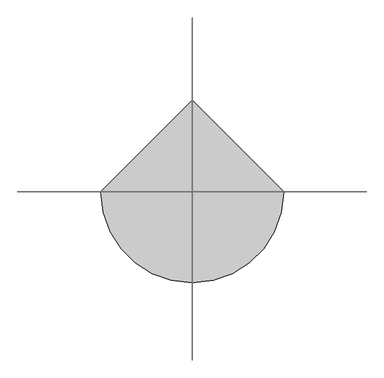
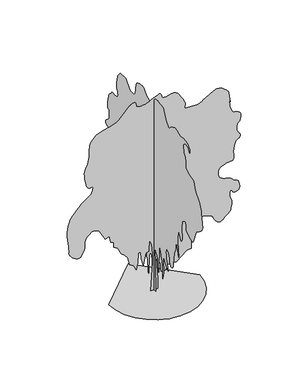
"""IFC4 building model written with IfcOpenShell, lengths in millimetres: geographic element geometry, RPC 木 - 落葉樹 : キングサリ - 5.5 メートル."""

from ifc_helpers import new_model, si_unit, origin, place, context, project, spatial, triangles, source, transform, mapped, element, save


def geographic_element_a00e3d8d(model_context):
    return source(origin(), model_context, "Body", "Tessellation", [
        triangles([(-0.0021492, 84.2526244, 0.0017055), (-0.0021492, -79.7118133, 0.0017055), (-0.0021492, -55.1171344, 770.634066), (-0.0021492, -30.52271, 1205.1392303), (-0.0021492, -128.9011709, 1090.3649134), (-0.0021492, -161.6941638, 983.7871164), (-0.0021492, -161.6941638, 778.8331295), (-0.0021492, -202.6851937, 614.866975), (-0.0021492, -227.2798771, 1410.0957607), (-0.0021492, -292.8648455, 1254.3285244), (-0.0021492, -391.2435608, 934.5977497), (-0.0021492, -407.6416878, 557.4810519), (-0.0021492, -448.631991, 754.2384825), (-0.0021492, -424.0373076, 1123.1586239), (-0.0021492, -399.4426243, 1229.73395), (-0.0021492, -563.406308, 1024.7799631), (-0.0021492, -645.3893852, 910.0031027), (-0.0021492, -571.6053715, 1164.1489271), (-0.0021492, -566.3701896, 1202.7023878), (-0.0021492, -561.3514189, 1240.6803749), (-0.0021492, -556.7629998, 1277.5125744), (-0.0021492, -552.8188002, 1312.6235126), (-0.0021492, -549.7352311, 1345.4427303), (-0.0021492, -547.7261968, 1375.3897396), (-0.0021492, -547.0106881, 1401.8966972), (-0.0021492, -548.2049103, 1425.0577835), (-0.0021492, -551.5507453, 1445.6369053), (-0.0021492, -556.6891671, 1464.0644142), (-0.0021492, -563.2636931, 1480.7706619), (-0.0021492, -570.9127902, 1496.1886162), (-0.0021492, -579.2773596, 1510.7457218), (-0.0021492, -588.000955, 1524.870005), (-0.0021492, -615.9185823, 1493.2475166), (-0.0021492, -642.6878059, 1461.6276443), (-0.0021492, -667.1627655, 1430.0051559), (-0.0021492, -688.1977461, 1398.3828129), (-0.0021492, -704.6417278, 1366.7627953), (-0.0021492, -715.3489231, 1335.1404522), (-0.0021492, -719.1734716, 1303.5179638), (-0.0021492, -720.8463346, 1273.0922047), (-0.0021492, -725.5315138, 1244.8155876), (-0.0021492, -732.7248247, 1218.3341372), (-0.0021492, -741.92717, 1193.2836313), (-0.0021492, -752.6342926, 1169.3103127), (-0.0021492, -764.3473131, 1146.0549734), (-0.0021492, -776.5592857, 1123.1586239), (-0.0021492, -799.2416948, 1123.4208899), (-0.0021492, -820.9921841, 1125.2619112), (-0.0021492, -840.8787609, 1130.2577545), (-0.0021492, -857.9695055, 1139.9845591), (-0.0021492, -871.3299545, 1156.0211529), (-0.0021492, -880.0306589, 1179.9486895), (-0.0021492, -883.1370827, 1213.3382938), (-0.0021492, -884.8100183, 1255.5711811), (-0.0021492, -889.4951975, 1304.2589069), (-0.0021492, -896.6885084, 1358.3243568), (-0.0021492, -905.890781, 1416.6931778), (-0.0021492, -916.5979763, 1478.2854939), (-0.0021492, -928.3109241, 1542.0320389), (-0.0021492, -940.5255129, 1606.8530823), (-0.0021492, -1006.1104631, 1762.6177025), (-0.0021492, -1030.7051828, 2041.3582466), (-0.0021492, -1137.2829798, 1615.049675), (-0.0021492, -1096.2901331, 2033.1591831), (-0.0021492, -1120.8847801, 2385.683741), (-0.0021492, -1260.2563602, 2139.7369801), (-0.0021492, -1270.7241806, 2153.8612633), (-0.0021492, -1280.7616493, 2168.4185143), (-0.0021492, -1289.9410309, 2183.833707), (-0.0021492, -1297.8295029, 2200.5425709), (-0.0021492, -1303.9940975, 2218.9700798), (-0.0021492, -1308.0095501, 2239.5492016), (-0.0021492, -1309.4456543, 2262.7104332), (-0.0021492, -1307.6275967, 2290.0779488), (-0.0021492, -1302.9424175, 2322.0339924), (-0.0021492, -1296.5385933, 2357.1449306), (-0.0021492, -1289.5590775, 2393.9769848), (-0.0021492, -1283.1526371, 2431.0969574), (-0.0021492, -1278.467458, 2467.0685989), (-0.0021492, -1276.6520164, 2500.4581306), (-0.0021492, -1277.8461296, 2532.7959824), (-0.0021492, -1281.1946171, 2566.4378242), (-0.0021492, -1286.3329662, 2601.1438454), (-0.0021492, -1292.9049488, 2636.6899315), (-0.0021492, -1300.5540459, 2672.8984772), (-0.0021492, -1308.9186516, 2709.5395546), (-0.0021492, -1317.642247, 2746.4099785), (-0.0021492, -1349.0965771, 2763.5973015), (-0.0021492, -1379.5477707, 2778.4931946), (-0.0021492, -1407.98993, 2788.7803574), (-0.0021492, -1433.4223892, 2792.1923584), (-0.0021492, -1454.8366344, 2786.4377678), (-0.0021492, -1471.2349068, 2769.1992851), (-0.0021492, -1481.6059307, 2738.2107697), (-0.0021492, -1484.4043064, 2701.9007767), (-0.0021492, -1481.8937038, 2669.6135033), (-0.0021492, -1478.8100258, 2640.331279), (-0.0021492, -1479.8871403, 2613.0602692), (-0.0021492, -1489.8533924, 2586.7825127), (-0.0021492, -1513.4448303, 2560.530336), (-0.0021492, -1555.3924152, 2533.2517685), (-0.0021492, -1606.8990097, 2505.0720932), (-0.0021492, -1655.2531803, 2478.4681938), (-0.0021492, -1699.3015091, 2456.025087), (-0.0021492, -1737.903368, 2440.3222664), (-0.0021492, -1769.9078098, 2433.9411152), (-0.0021492, -1794.1663582, 2439.4615631), (-0.0021492, -1809.5357689, 2459.4679001), (-0.0021492, -1957.1037964, 2820.1761154), (-0.0021492, -2096.4729057, 2918.565168), (-0.0021492, -2133.9034698, 2947.2108032), (-0.0021492, -2168.0339447, 2976.9770096), (-0.0021492, -2197.5760368, 3008.067263), (-0.0021492, -2221.2388367, 3040.5580124), (-0.0021492, -2237.731144, 3074.6530243), (-0.0021492, -2245.7621944, 3110.4540367), (-0.0021492, -2244.0409332, 3148.1136566), (-0.0021492, -2235.2459759, 3194.9401588), (-0.0021492, -2223.8691994, 3254.6760475), (-0.0021492, -2211.3439465, 3322.1530334), (-0.0021492, -2199.1064667, 3392.2016647), (-0.0021492, -2188.5902481, 3459.6786507), (-0.0021492, -2181.2289242, 3519.4145393), (-0.0021492, -2178.455983, 3566.2154617), (-0.0021492, -2170.3281361, 3608.6878693), (-0.0021492, -2147.5744377, 3658.060437), (-0.0021492, -2112.6316578, 3713.1367264), (-0.0021492, -2067.93395, 3772.8220367), (-0.0021492, -2015.9257874, 3835.9446373), (-0.0021492, -1959.038998, 3901.3845383), (-0.0021492, -1899.7154388, 3967.9447197), (-0.0021492, -1842.3295521, 4197.493499), (-0.0021492, -1629.1739582, 4246.6878799), (-0.0021492, -1457.0138271, 4328.6532257), (-0.0021492, -1458.3505188, 4335.1970123), (-0.0021492, -1461.6963902, 4352.7409996), (-0.0021492, -1466.0480141, 4378.3568779), (-0.0021492, -1470.3971672, 4408.9634399), (-0.0021492, -1473.7428932, 4441.6067963), (-0.0021492, -1475.0823463, 4473.206321), (-0.0021492, -1473.409338, 4500.8337044), (-0.0021492, -1467.7438408, 4526.8568253), (-0.0021492, -1458.2079403, 4555.4518822), (-0.0021492, -1445.4434578, 4586.2110512), (-0.0021492, -1430.0994816, 4618.7018005), (-0.0021492, -1412.8176876, 4652.465728), (-0.0021492, -1394.2476002, 4687.1208801), (-0.0021492, -1375.0306046, 4722.1832748), (-0.0021492, -1342.2369667, 4918.9358002), (-0.0021492, -1448.8147636, 5009.1256439), (-0.0021492, -1579.9871349, 4984.5283081), (-0.0021492, -1653.7686779, 4877.9400467), (-0.0021492, -1653.7686779, 4976.32939), (-0.0021492, -1538.9942883, 5082.8914902), (-0.0021492, -1350.4360302, 5107.488826), (-0.0021492, -1202.86793, 5074.692572), (-0.0021492, -1055.2998299, 5156.6834976), (-0.0021492, -948.7220329, 5164.8824158), (-0.0021492, -940.8820318, 5161.1390396), (-0.0021492, -920.1373678, 5151.1070938), (-0.0021492, -890.6410578, 5136.4911255), (-0.0021492, -856.5588358, 5118.9980072), (-0.0021492, -822.0437914, 5100.3340302), (-0.0021492, -791.2591152, 5082.280481), (-0.0021492, -768.3627657, 5066.4936539), (-0.0021492, -752.5401123, 5050.8591431), (-0.0021492, -739.1542288, 5033.7991379), (-0.0021492, -726.6289759, 5017.8844116), (-0.0021492, -713.388287, 5005.688063), (-0.0021492, -697.8532614, 4999.805864), (-0.0021492, -678.4454344, 5002.8359116), (-0.0021492, -653.5859053, 5017.2989822), (-0.0021492, -627.152853, 5039.5790176), (-0.0021492, -603.7294644, 5064.0234558), (-0.0021492, -582.8141713, 5090.2247635), (-0.0021492, -563.9079125, 5117.8777267), (-0.0021492, -546.5090836, 5146.6253906), (-0.0021492, -530.1109202, 5176.0608032), (-0.0021492, -514.2169413, 5205.8775879), (-0.0021492, -415.8382442, 5410.8290314), (-0.0021492, -169.8924643, 5451.8247849), (-0.0021492, -163.845268, 5451.6718872), (-0.0021492, -147.6161895, 5450.6789246), (-0.0021492, -124.0728773, 5447.9540909), (-0.0021492, -96.0842423, 5442.6323227), (-0.0021492, -66.5181782, 5433.8985535), (-0.0021492, -38.242574, 5420.8359787), (-0.0021492, -14.1260636, 5402.6301132), (-0.0021492, 3.3458591, 5384.2457703), (-0.0021492, 15.2248417, 5370.0373352), (-0.0021492, 23.9488607, 5358.0956223), (-0.0021492, 31.9557666, 5346.6114395), (-0.0021492, 41.6836385, 5333.6761826), (-0.0021492, 55.5706315, 5317.4312439), (-0.0021492, 76.0543103, 5296.0418518), (-0.0021492, 97.1353591, 5271.2921997), (-0.0021492, 113.1971422, 5247.5349289), (-0.0021492, 127.251426, 5226.7827072), (-0.0021492, 142.3092006, 5211.0464584), (-0.0021492, 161.3827366, 5202.3638489), (-0.0021492, 187.4830512, 5202.6946426), (-0.0021492, 223.6221243, 5214.0770874), (-0.0021492, 264.3514152, 5233.7851868), (-0.0021492, 302.4974698, 5257.3895599), (-0.0021492, 338.4919115, 5284.2018768), (-0.0021492, 372.7676173, 5313.5861298), (-0.0021492, 405.7523409, 5344.9307281), (-0.0021492, 437.8764338, 5377.549086), (-0.0021492, 469.5676317, 5410.8290314), (-0.0021492, 492.4664884, 5419.4866425), (-0.0021492, 515.7217913, 5427.329187), (-0.0021492, 539.6951826, 5433.618338), (-0.0021492, 564.7456521, 5437.5396103), (-0.0021492, 591.2271389, 5438.3035172), (-0.0021492, 619.503756, 5435.1205719), (-0.0021492, 649.9294424, 5427.227449), (-0.0021492, 681.4067362, 5417.9076691), (-0.0021492, 712.0260155, 5409.8616486), (-0.0021492, 740.9213448, 5401.4080948), (-0.0021492, 767.2373257, 5390.7895569), (-0.0021492, 790.1107115, 5376.3014877), (-0.0021492, 808.683415, 5356.2364334), (-0.0021492, 822.0921896, 5328.8381058), (-0.0021492, 831.6764883, 5297.4679276), (-0.0021492, 839.5394531, 5266.5052826), (-0.0021492, 845.9687845, 5235.9240097), (-0.0021492, 851.252401, 5205.5973724), (-0.0021492, 855.6727707, 5175.5259521), (-0.0021492, 859.5227537, 5145.5556885), (-0.0021492, 863.0824928, 5115.6877441), (-0.0021492, 868.5086151, 5085.9982773), (-0.0021492, 874.8667299, 5057.4029297), (-0.0021492, 883.0887571, 5030.9469864), (-0.0021492, 894.1065439, 5007.6995682), (-0.0021492, 908.8546989, 4988.7803741), (-0.0021492, 928.2625986, 4975.2085281), (-0.0021492, 953.2646336, 4968.1298904), (-0.0021492, 983.5707052, 4964.7946289), (-0.0021492, 1017.0341423, 4962.6302261), (-0.0021492, 1051.7859455, 4962.7319641), (-0.0021492, 1085.9648912, 4966.2968628), (-0.0021492, 1117.7070671, 4974.4446213), (-0.0021492, 1145.1459446, 4988.3478424), (-0.0021492, 1166.417684, 5009.1256439), (-0.0021492, 1187.9516893, 5037.6186722), (-0.0021492, 1215.2250973, 5071.5857849), (-0.0021492, 1244.9327316, 5107.4126678), (-0.0021492, 1273.7822788, 5141.5326782), (-0.0021492, 1298.4736496, 5170.3315018), (-0.0021492, 1315.7070454, 5190.2436584), (-0.0021492, 1322.1822315, 5197.6786697), (-0.0021492, 1576.3282013, 5181.2802521), (-0.0021492, 1674.7067894, 5058.2941544), (-0.0021492, 1679.9878624, 5049.3057495), (-0.0021492, 1685.3427681, 5039.1209061), (-0.0021492, 1690.8402523, 5026.4658646), (-0.0021492, 1696.5540024, 5010.1691849), (-0.0021492, 1702.550584, 4988.9844315), (-0.0021492, 1708.9087715, 4961.7134216), (-0.0021492, 1715.6971653, 4927.1347183), (-0.0021492, 1722.2461842, 4888.9655365), (-0.0021492, 1727.9346451, 4851.6622902), (-0.0021492, 1732.9075974, 4815.0467926), (-0.0021492, 1737.3050034, 4779.0420135), (-0.0021492, 1741.2720577, 4743.4447678), (-0.0021492, 1744.9541004, 4708.1530266), (-0.0021492, 1748.4909485, 4672.9888939), (-0.0021492, 1731.0895397, 4648.3406891), (-0.0021492, 1714.6938835, 4623.4122688), (-0.0021492, 1700.3047909, 4597.923999), (-0.0021492, 1688.927869, 4571.5442139), (-0.0021492, 1681.5665451, 4544.0444389), (-0.0021492, 1679.2239555, 4515.0930084), (-0.0021492, 1682.9058529, 4484.4355774), (-0.0021492, 1691.9172215, 4457.546521), (-0.0021492, 1704.7989933, 4438.9587021), (-0.0021492, 1721.4110607, 4426.9911186), (-0.0021492, 1741.6082291, 4419.8869011), (-0.0021492, 1765.2454491, 4415.940049), (-0.0021492, 1792.1827583, 4413.4448524), (-0.0021492, 1822.2749622, 4410.6438606), (-0.0021492, 1851.5776794, 4410.5165428), (-0.0021492, 1877.0101387, 4414.7180305), (-0.0021492, 1899.7154388, 4419.4540787), (-0.0021492, 1920.8445271, 4421.0583412), (-0.0021492, 1941.543409, 4415.787442), (-0.0021492, 1962.9577995, 4399.8985863), (-0.0021492, 1986.2386459, 4369.6483978), (-0.0021492, 2009.8529022, 4339.0165466), (-0.0021492, 2031.6034641, 4320.2758301), (-0.0021492, 2051.6326195, 4307.2641243), (-0.0021492, 2070.0855629, 4293.8451759), (-0.0021492, 2087.1025475, 4273.8059921), (-0.0021492, 2102.8309479, 4241.0097382), (-0.0021492, 2117.4110172, 4189.2942902), (-0.0021492, 2130.4608021, 4132.1300468), (-0.0021492, 2141.5041687, 4085.4564423), (-0.0021492, 2150.5383556, 4046.6762512), (-0.0021492, 2157.5661243, 4013.1925392), (-0.0021492, 2162.5848587, 3982.4330795), (-0.0021492, 2165.5945587, 3951.8012283), (-0.0021492, 2166.6004566, 3918.7503387), (-0.0021492, 2163.9700939, 3888.1437767), (-0.0021492, 2156.60877, 3865.7364235), (-0.0021492, 2145.3032101, 3850.1274925), (-0.0021492, 2130.8427555, 3839.9679382), (-0.0021492, 2114.016893, 3833.907843), (-0.0021492, 2095.6122025, 3830.546711), (-0.0021492, 2076.4181705, 3828.560495), (-0.0021492, 2076.4181705, 3615.4101334), (-0.0021492, 2076.5863289, 3611.7687859), (-0.0021492, 2077.7576237, 3607.2365044), (-0.0021492, 2080.9353367, 3600.9979317), (-0.0021492, 2087.1279819, 3592.1877136), (-0.0021492, 2097.3334637, 3579.9146255), (-0.0021492, 2112.5578251, 3563.3636009), (-0.0021492, 2133.8066734, 3541.6437057), (-0.0021492, 2158.6890209, 3518.82911), (-0.0021492, 2183.2837406, 3498.7640556), (-0.0021492, 2206.2997776, 3480.0997879), (-0.0021492, 2226.4485477, 3461.613707), (-0.0021492, 2242.4392868, 3441.9561859), (-0.0021492, 2252.9809399, 3419.8799171), (-0.0021492, 2256.7799812, 3394.0605629), (-0.0021492, 2250.3277588, 3369.7687317), (-0.0021492, 2232.2566235, 3352.3776421), (-0.0021492, 2204.5071545, 3340.7155632), (-0.0021492, 2169.0142628, 3333.6369255), (-0.0021492, 2127.7108246, 3329.995578), (-0.0021492, 2082.5369831, 3328.6715309), (-0.0021492, 2035.42794, 3328.4677643), (-0.0021492, 2021.5658501, 3329.995578), (-0.0021492, 2008.8497658, 3330.1737648), (-0.0021492, 1998.4277275, 3327.6276993), (-0.0021492, 1991.4508278, 3320.981884), (-0.0021492, 1989.05984, 3308.8869827), (-0.0021492, 1992.4057114, 3289.9677887), (-0.0021492, 2002.6367729, 3262.9008362), (-0.0021492, 2020.3945553, 3234.9679482), (-0.0021492, 2044.3195484, 3213.2224731), (-0.0021492, 2072.5479126, 3195.7802238), (-0.0021492, 2103.2129013, 3180.7573036), (-0.0021492, 2134.4508202, 3166.3198128), (-0.0021492, 2164.4004456, 3150.6091438), (-0.0021492, 2191.195031, 3131.7155296), (-0.0021492, 2214.6668541, 3115.4703003), (-0.0021492, 2235.4115181, 3106.0996513), (-0.0021492, 2252.7161304, 3099.4538361), (-0.0021492, 2265.8627117, 3091.3822357), (-0.0021492, 2274.1329918, 3077.7086517), (-0.0021492, 2276.8092819, 3054.282756), (-0.0021492, 2273.1756374, 3016.9539299), (-0.0021492, 2263.7594971, 2975.5765137), (-0.0021492, 2250.0399857, 2941.9401947), (-0.0021492, 2232.7353733, 2914.7709229), (-0.0021492, 2212.5636395, 2892.7455231), (-0.0021492, 2190.2376766, 2874.6161064), (-0.0021492, 2166.4806965, 2859.0580444), (-0.0021492, 2142.0057369, 2844.7734512), (-0.0021492, 2133.3763218, 2827.178595), (-0.0021492, 2125.6814426, 2809.2779434), (-0.0021492, 2119.8477871, 2790.7918625), (-0.0021492, 2116.8126526, 2771.4654259), (-0.0021492, 2117.5051975, 2750.9678398), (-0.0021492, 2122.8601032, 2729.044178), (-0.0021492, 2133.8066734, 2705.4145157), (-0.0021492, 2153.6932503, 2682.9815826), (-0.0021492, 2182.4714355, 2663.4008011), (-0.0021492, 2215.9807274, 2644.532476), (-0.0021492, 2250.0629494, 2624.2386566), (-0.0021492, 2280.5623959, 2600.3543587), (-0.0021492, 2303.3160942, 2570.74105), (-0.0021492, 2314.1684841, 2533.2517685), (-0.0021492, 2316.6306885, 2491.7827881), (-0.0021492, 2316.7962307, 2450.4565315), (-0.0021492, 2314.3824245, 2407.4087231), (-0.0021492, 2309.1013515, 2360.7784298), (-0.0021492, 2300.6629131, 2308.6964344), (-0.0021492, 2288.7844231, 2249.3015133), (-0.0021492, 2273.1756374, 2180.7272106), (-0.0021492, 2256.9481396, 2122.3126076), (-0.0021492, 2242.7270599, 2087.8459614), (-0.0021492, 2229.5092621, 2067.1472248), (-0.0021492, 2216.2913189, 2050.0334438), (-0.0021492, 2202.0703846, 2026.3248619), (-0.0021492, 2185.8402706, 1985.8337288), (-0.0021492, 2166.6004566, 1918.3849388), (-0.0021492, 2149.5810013, 1842.5205288), (-0.0021492, 2138.873806, 1783.2936207), (-0.0021492, 2131.751857, 1740.2713921), (-0.0021492, 2125.4904659, 1713.0234913), (-0.0021492, 2117.362619, 1701.1195667), (-0.0021492, 2104.6465347, 1704.1318829), (-0.0021492, 2084.617234, 1721.6274719), (-0.0021492, 2060.5012642, 1758.077718), (-0.0021492, 2037.2459976, 1813.4570412), (-0.0021492, 2014.7062397, 1880.5978558), (-0.0021492, 1992.7392666, 1952.324437), (-0.0021492, 1971.2052612, 2021.4716698), (-0.0021492, 1949.9564129, 2080.8665909), (-0.0021492, 1928.8527592, 2123.3388531), (-0.0021492, 1903.2293232, 2154.4825916), (-0.0021492, 1869.4322582, 2184.768243), (-0.0021492, 1828.8239811, 2214.3332989), (-0.0021492, 1782.766618, 2243.3254246), (-0.0021492, 1732.6198242, 2271.8871986), (-0.0021492, 1679.7511036, 2300.1638157), (-0.0021492, 1625.5174953, 2328.2953835), (-0.0021492, 1580.1042789, 2357.6694626), (-0.0021492, 1536.2697453, 2384.1050583), (-0.0021492, 1495.5901062, 2404.6613617), (-0.0021492, 1459.6415737, 2416.3971279), (-0.0021492, 1430.0026852, 2416.3716934), (-0.0021492, 1408.2522686, 2401.6490456), (-0.0021492, 1395.9662453, 2369.285614), (-0.0021492, 1387.7443634, 2327.3633183), (-0.0021492, 1377.3731941, 2285.8715195), (-0.0021492, 1365.2070763, 2244.7360943), (-0.0021492, 1351.607325, 2203.8884422), (-0.0021492, 1336.9304592, 2163.2545853), (-0.0021492, 1321.5380848, 2122.7659229), (-0.0021492, 1305.7867207, 2082.3484772), (-0.0021492, 1125.4248373, 1926.5840023), (-0.0021492, 1107.9776464, 1907.1276318), (-0.0021492, 1091.2458916, 1886.8820652), (-0.0021492, 1075.9503136, 1865.0602867), (-0.0021492, 1062.803805, 1840.8731003), (-0.0021492, 1052.5269613, 1813.5284031), (-0.0021492, 1045.8352913, 1782.242086), (-0.0021492, 1043.4443035, 1746.2221916), (-0.0021492, 1042.7262514, 1711.1596516), (-0.0021492, 1040.7197605, 1682.5468632), (-0.0021492, 1037.6362278, 1659.3170311), (-0.0021492, 1033.6919918, 1640.3853378), (-0.0021492, 1029.1035364, 1624.6823719), (-0.0021492, 1024.0848021, 1611.1308735), (-0.0021492, 1018.8495838, 1598.6540188), (-0.0021492, 871.2815563, 1500.2752853), (-0.0021492, 854.8859728, 1328.1125381), (-0.0021492, 731.9125923, 1270.7241806), (-0.0021492, 699.1188091, 1057.5711302), (-0.0021492, 567.9463288, 1024.7799631), (-0.0021492, 579.9928682, 1019.3537682), (-0.0021492, 590.5345213, 1012.9956533), (-0.0021492, 598.0639309, 1004.7736988), (-0.0021492, 601.0736672, 993.7558393), (-0.0021492, 598.0639309, 979.0076843), (-0.0021492, 587.5222778, 959.5998573), (-0.0021492, 567.9463288, 934.5977497), (-0.0021492, 544.3090725, 908.8801334), (-0.0021492, 522.3905339, 887.4632721), (-0.0021492, 501.9081359, 869.6341278), (-0.0021492, 482.5715618, 854.6720324), (-0.0021492, 464.0956547, 841.8616224), (-0.0021492, 446.1926414, 830.4822298), (-0.0021492, 428.5773648, 819.8234327), (-0.0021492, 416.3169213, 852.4975285), (-0.0021492, 404.2704183, 880.9396877), (-0.0021492, 392.6541942, 900.9204449), (-0.0021492, 381.6821895, 908.2104795), (-0.0021492, 371.5733952, 898.5778553), (-0.0021492, 362.5365921, 867.7931065), (-0.0021492, 354.7933147, 811.6243692), (-0.0021492, 347.289376, 757.5588467), (-0.0021492, 338.9222631, 728.4470335), (-0.0021492, 329.8396053, 713.1030573), (-0.0021492, 320.1840537, 700.3410456), (-0.0021492, 310.0981868, 678.9725098), (-0.0021492, 299.7245649, 637.8141935), (-0.0021492, 289.2083645, 565.6776083), (-0.0021492, 280.100254, 485.3215756), (-0.0021492, 273.5766333, 424.7553597), (-0.0021492, 269.2021002, 380.6815238), (-0.0021492, 266.5488646, 349.8000149), (-0.0021492, 265.1865931, 328.8160123), (-0.0021492, 264.6849704, 314.4268833), (-0.0021492, 264.6136811, 303.3352093), (-0.0021492, 240.0187434, 811.6243692), (-0.0021492, 227.6618305, 844.6574547), (-0.0021492, 214.9461277, 875.6102892), (-0.0021492, 201.5133903, 902.4024038), (-0.0021492, 187.005355, 922.9586346), (-0.0021492, 171.062996, 935.1961143), (-0.0021492, 153.3280502, 937.0371357), (-0.0021492, 133.441982, 926.4012297), (-0.0021492, 115.7070271, 904.2917507), (-0.0021492, 103.9950785, 874.0086428), (-0.0021492, 97.3026454, 836.9141773), (-0.0021492, 94.6257285, 794.3681551), (-0.0021492, 94.9603102, 747.7377892), (-0.0021492, 97.3026454, 698.3804094), (-0.0021492, 100.6487348, 647.6606855), (-0.0021492, 84.2526244, 237.7500047), (88.443575, 0.0002505, 0.0), (-86.3932913, 0.0002505, 0.0), (-44.7656769, 0.0002025, 807.5808661), (-36.4400495, 0.0001919, 1032.3704882), (-69.7422955, 0.0001759, 1307.1158546), (-128.0216733, 0.0001652, 1448.6492214), (-144.6726737, 0.0001865, 1140.603344), (-227.9279117, 0.0001865, 1115.6267435), (-294.532658, 0.0002025, 799.2544847), (-352.8122947, 0.0001919, 999.0699772), (-361.138676, 0.0001812, 1182.2301636), (-427.7421687, 0.0001812, 1182.2301636), (-444.3923879, 0.0001972, 915.8137218), (-486.0217873, 0.0002079, 732.650992), (-552.62528, 0.0002025, 874.1843588), (-660.8581358, 0.0001972, 940.7903223), (-702.4850281, 0.0001812, 1157.2535631), (-785.7412834, 0.0001759, 1257.1626537), (-877.3239201, 0.0001759, 1332.0925278), (-977.2303946, 0.0001599, 1523.5790955), (-1085.4632504, 0.0001599, 1581.8586777), (-1085.4632504, 0.0001492, 1723.3945152), (-1160.3931244, 0.0001492, 1748.3711884), (-1202.0200167, 0.0001386, 1939.857756), (-1318.5792538, 0.0001386, 1889.9045551), (-1468.4390018, 0.0001226, 2172.9737595), (-1502.3251602, 0.0001226, 2194.044421), (-1536.1348698, 0.0001226, 2213.0729107), (-1569.8020008, 0.0001173, 2228.0247597), (-1603.2501045, 0.0001173, 2236.8604122), (-1636.4054935, 0.0001173, 2237.5401672), (-1669.1992767, 0.0001173, 2228.0247597), (-1701.5550053, 0.0001226, 2206.2768139), (-1733.4728245, 0.0001226, 2179.0187393), (-1764.2270519, 0.0001226, 2153.3621658), (-1792.6513344, 0.0001279, 2127.8509323), (-1817.5796093, 0.0001279, 2101.0307671), (-1837.8479942, 0.0001279, 2071.4427475), (-1852.2881012, 0.0001332, 2037.6304218), (-1859.7411346, 0.0001332, 1998.1374836), (-1862.0709343, 0.0001386, 1954.9318359), (-1863.0894768, 0.0001386, 1911.4360897), (-1864.5459286, 0.0001439, 1868.3756367), (-1868.1871307, 0.0001439, 1826.4813915), (-1875.7599243, 0.0001439, 1786.4790367), (-1889.0133305, 0.0001492, 1749.0994869), (-1909.6943356, 0.0001492, 1715.0681339), (-1930.6657299, 0.0001546, 1683.7079842), (-1945.9586918, 0.0001546, 1654.8228287), (-1959.0645779, 0.0001546, 1629.87159), (-1973.4841919, 0.0001546, 1610.3059238), (-1992.7087452, 0.0001599, 1597.5872234), (-2020.2342453, 0.0001599, 1593.1693245), (-2059.5540836, 0.0001599, 1598.5089695), (-2106.0851097, 0.0001546, 1614.4818317), (-2151.452544, 0.0001546, 1639.629134), (-2193.466404, 0.0001546, 1671.9110298), (-2229.9497875, 0.0001492, 1709.2905796), (-2258.7127121, 0.0001492, 1749.7309891), (-2277.5730434, 0.0001439, 1791.1871796), (-2284.3437057, 0.0001439, 1831.6274437), (-2284.0050636, 0.0001439, 1867.2348633), (-2283.6664215, 0.0001386, 1899.3462753), (-2284.3437057, 0.0001386, 1933.6447632), (-2287.0631618, 0.0001332, 1975.8064339), (-2292.8407162, 0.0001332, 2031.5117546), (-2302.6949112, 0.0001279, 2106.4440994), (-2317.6467602, 0.0001226, 2206.2768139), (-2328.3767738, 0.0001119, 2318.4666229), (-2327.0171185, 0.0001066, 2424.8304794), (-2316.773267, 0.0001013, 2522.6006744), (-2300.8512737, 9.59e-05, 2609.0116791), (-2282.4518154, 9.06e-05, 2681.301162), (-2264.7805103, 9.06e-05, 2736.6829559), (-2251.0432674, 8.53e-05, 2772.4075195), (-2228.7606159, 8.53e-05, 2807.0373825), (-2187.9817097, 7.99e-05, 2856.639006), (-2135.6985638, 7.99e-05, 2914.8473717), (-2078.9008678, 7.46e-05, 2975.2457199), (-2024.5781662, 7.46e-05, 3031.4170006), (-1979.7200031, 6.93e-05, 3076.9447449), (-1951.3211552, 6.93e-05, 3105.4377731), (-1924.2821079, 6.4e-05, 3127.0812195), (-1882.8233013, 6.4e-05, 3155.294323), (-1832.9184986, 6.4e-05, 3188.4469505), (-1780.5385563, 5.86e-05, 3224.9610008), (-1731.6521507, 5.86e-05, 3263.2063408), (-1692.2330452, 5.33e-05, 3301.6042877), (-1668.2519508, 5.33e-05, 3338.5511604), (-1656.1647526, 5.33e-05, 3371.3221252), (-1648.0090004, 4.8e-05, 3398.84748), (-1643.1302284, 4.8e-05, 3421.9934509), (-1640.8716454, 4.8e-05, 3441.6762611), (-1640.5814014, 4.8e-05, 3458.7109772), (-1641.5999439, 4.8e-05, 3473.9888237), (-1643.275423, 4.26e-05, 3488.4263145), (-1673.4947994, 4.26e-05, 3483.4864998), (-1703.0598553, 4.26e-05, 3481.1183304), (-1731.3135086, 4.26e-05, 3483.8172935), (-1757.6015842, 4.26e-05, 3494.1809052), (-1781.2668549, 4.26e-05, 3514.75494), (-1801.657616, 4.26e-05, 3548.0604652), (-1818.114315, 3.73e-05, 3596.643837), (-1832.6281094, 3.2e-05, 3658.2386238), (-1846.5615612, 3.2e-05, 3726.3521988), (-1858.3075012, 2.66e-05, 3797.4193726), (-1866.2698059, 2.13e-05, 3867.7226395), (-1868.8440674, 1.6e-05, 3933.671521), (-1864.4263138, 1.6e-05, 3991.625251), (-1851.4147533, 1.07e-05, 4037.891613), (-1831.8515579, 1.07e-05, 4080.6183655), (-1810.1036121, 5.3e-06, 4129.8891953), (-1788.0628063, 5.3e-06, 4185.1439621), (-1767.626263, 0.0, 4245.7710754), (-1750.6832565, -5.3e-06, 4311.2109764), (-1739.1281479, -1.07e-05, 4380.8776543), (-1734.8580597, -1.07e-05, 4454.1856796), (-1735.4895618, -1.6e-05, 4523.8776466), (-1735.828204, -2.13e-05, 4584.5303398), (-1733.5466572, -2.13e-05, 4638.3337418), (-1726.3126511, -2.66e-05, 4687.5028336), (-1711.7987114, -3.2e-05, 4734.1764381), (-1687.670097, -3.2e-05, 4780.5442474), (-1651.6018044, -3.73e-05, 4828.8221146), (-1604.6581581, -3.73e-05, 4875.2410835), (-1551.3057461, -4.26e-05, 4914.6575729), (-1494.3144573, -4.26e-05, 4947.2247711), (-1436.4473499, -4.26e-05, 4973.1208649), (-1380.4746037, -4.26e-05, 4992.421431), (-1329.1617474, -4.8e-05, 5005.3566879), (-1285.2761993, -4.8e-05, 5012.0027939), (-1238.8191513, -4.8e-05, 5019.8197586), (-1181.7285954, -4.8e-05, 5034.7665207), (-1119.6855074, -4.8e-05, 5054.8059952), (-1058.3732615, -4.8e-05, 5077.9260956), (-1003.4674559, -5.33e-05, 5102.03974), (-960.6514647, -5.33e-05, 5125.1604218), (-935.6010315, -5.33e-05, 5145.1993149), (-669.1845171, -6.93e-05, 5428.27099), (-646.0030832, -6.93e-05, 5444.1601364), (-622.8954094, -7.46e-05, 5458.928421), (-599.9329302, -7.46e-05, 5471.5328842), (-577.1894056, -7.46e-05, 5480.8520828), (-554.7387048, -7.46e-05, 5485.7918976), (-532.6495734, -7.46e-05, 5485.2826263), (-510.9984241, -7.46e-05, 5478.2295685), (-495.8275841, -7.46e-05, 5462.4933197), (-489.5407948, -6.93e-05, 5439.0418442), (-486.7500495, -6.93e-05, 5411.3894623), (-482.0648704, -6.93e-05, 5382.9725922), (-470.0972506, -6.93e-05, 5357.3567139), (-445.4618357, -6.4e-05, 5337.9794083), (-402.7655319, -6.4e-05, 5328.3544144), (-352.155358, -6.4e-05, 5326.9794983), (-306.7905398, -6.4e-05, 5329.5258545), (-265.7951679, -6.4e-05, 5335.3568939), (-228.2925333, -6.4e-05, 5343.8104477), (-193.4123586, -6.4e-05, 5354.2249283), (-160.2802058, -6.93e-05, 5365.9381668), (-128.0216733, -6.93e-05, 5378.3129929), (-76.4902348, -6.93e-05, 5408.3594147), (-26.1968067, -6.93e-05, 5436.750705), (21.6206802, -7.46e-05, 5461.7805725), (65.7244948, -7.46e-05, 5481.7688873), (104.8766017, -7.46e-05, 5495.0605179), (137.8389248, -7.46e-05, 5500.0003326), (163.3739486, -7.46e-05, 5494.8826218), (179.7578323, -7.46e-05, 5482.2525787), (188.4231464, -7.46e-05, 5466.2872742), (192.8648993, -7.46e-05, 5447.6994553), (196.5786806, -6.93e-05, 5427.2018692), (203.0594986, -6.93e-05, 5405.5584229), (215.802707, -6.93e-05, 5383.4562836), (238.3035683, -6.93e-05, 5361.6599396), (275.7078986, -6.4e-05, 5352.0099472), (327.5301169, -6.93e-05, 5359.8269119), (388.8194718, -6.93e-05, 5376.0974304), (454.6234131, -6.93e-05, 5391.7575211), (519.9894087, -6.93e-05, 5397.8431961), (579.9673974, -6.93e-05, 5385.2643127), (629.6048836, -6.4e-05, 5345.0074677), (669.510442, -6.4e-05, 5289.625383), (704.1732244, -5.86e-05, 5237.2989258), (734.4639627, -5.86e-05, 5187.5188248), (761.2611643, -5.33e-05, 5139.7758087), (785.4382496, -5.33e-05, 5093.5606064), (807.8660231, -4.8e-05, 5048.3639465), (829.4204487, -4.8e-05, 5003.6765579), (821.0940674, -3.73e-05, 4853.8014038), (1104.1632717, -3.73e-05, 4837.1486412), (1130.9121477, -3.73e-05, 4839.0836975), (1157.5871183, -3.73e-05, 4841.7826607), (1184.116967, -3.73e-05, 4846.1114662), (1210.4304045, -3.73e-05, 4852.8337303), (1236.4509819, -3.73e-05, 4862.7642288), (1262.1075554, -3.73e-05, 4876.6924484), (1287.3260742, -3.73e-05, 4895.433165), (1317.642247, -4.26e-05, 4918.5538467), (1357.5732399, -4.26e-05, 4944.7039948), (1405.5098488, -4.26e-05, 4973.4260788), (1459.8579849, -4.8e-05, 5004.1858292), (1519.0110603, -4.8e-05, 5036.4728119), (1581.3672832, -4.8e-05, 5069.7527573), (1645.3251526, -5.33e-05, 5103.5675537), (1684.4540142, -5.33e-05, 5099.8497574), (1722.8522518, -5.33e-05, 5095.2668976), (1759.7965084, -5.33e-05, 5088.9515854), (1794.5558693, -4.8e-05, 5079.9887604), (1826.3998558, -4.8e-05, 5067.5371948), (1854.6052563, -4.8e-05, 5050.7062454), (1878.441156, -4.8e-05, 5028.6552658), (1900.2145363, -4.8e-05, 5007.1902969), (1922.1329659, -4.26e-05, 4990.5372437), (1943.3232422, -4.26e-05, 4975.3358459), (1962.9120174, -4.26e-05, 4958.2502609), (1980.023037, -4.26e-05, 4935.9196472), (1993.7858597, -3.73e-05, 4905.0075806), (2003.3268471, -3.73e-05, 4862.1276398), (2036.6272854, -2.13e-05, 4620.6877258), (2031.3360386, -2.66e-05, 4643.2226875), (2026.4090137, -2.66e-05, 4661.7340576), (2022.2101421, -2.66e-05, 4672.2502762), (2019.1036457, -2.66e-05, 4670.7480423), (2017.4511303, -2.66e-05, 4653.2296349), (2017.6217594, -2.13e-05, 4615.6717529), (2019.9769936, -2.13e-05, 4554.0766754), (2029.0544918, -1.6e-05, 4483.8245682), (2046.7257969, -1.07e-05, 4423.1715843), (2069.3470905, -5.3e-06, 4372.5514183), (2093.2797867, -5.3e-06, 4332.4216003), (2114.8825378, -5.3e-06, 4303.241114), (2130.5142872, -5.3e-06, 4285.3916222), (2136.5336872, 0.0, 4279.3568161), (2147.5540901, 0.0, 4280.1463028), (2175.7594906, 0.0, 4279.6370316), (2213.8673389, 0.0, 4273.4493279), (2254.597847, 0.0, 4257.2040985), (2290.6661396, 0.0, 4226.5466675), (2314.7948994, 5.3e-06, 4177.0976509), (2319.6964897, 1.07e-05, 4104.5026634), (2308.0217663, 1.07e-05, 4035.0650414), (2289.5025478, 1.6e-05, 3991.3961952), (2267.4871765, 1.6e-05, 3963.6159142), (2245.3242851, 1.6e-05, 3941.794281), (2226.3696281, 2.13e-05, 3916.0257957), (2213.9641354, 2.13e-05, 3876.4308289), (2211.4661774, 2.66e-05, 3813.1044617), (2219.5964951, 2.66e-05, 3747.2826073), (2234.7189732, 3.2e-05, 3702.4170319), (2253.6252319, 3.2e-05, 3671.9886566), (2273.1170654, 3.73e-05, 3649.4284058), (2289.9862392, 3.73e-05, 3628.1416237), (2301.0320766, 3.73e-05, 3601.6601006), (2303.0461979, 4.26e-05, 3563.3383118), (2294.2843781, 4.26e-05, 3529.0395332), (2276.7837021, 4.26e-05, 3512.2341637), (2253.0191643, 4.26e-05, 3502.8382256), (2225.4708458, 4.26e-05, 3490.8197731), (2196.6085087, 4.8e-05, 3466.1206993), (2168.9149956, 4.8e-05, 3418.7340569), (2144.8600685, 5.33e-05, 3338.5511604), (2129.882785, 5.86e-05, 3243.8799042), (2124.958231, 6.4e-05, 3160.2850067), (2125.8545425, 6.93e-05, 3088.6321129), (2128.3549713, 7.46e-05, 3029.812738), (2128.2327404, 7.46e-05, 2984.6669472), (2121.2661598, 7.46e-05, 2954.085965), (2103.2332489, 7.99e-05, 2938.9354362), (2080.3674934, 7.99e-05, 2933.5627991), (2059.9793484, 7.99e-05, 2930.6853584), (2039.4433926, 7.99e-05, 2928.6482735), (2016.1423439, 7.99e-05, 2925.9237305), (1987.4506359, 7.99e-05, 2920.8565979), (1950.7508411, 7.99e-05, 2911.8429039), (1903.4176838, 7.99e-05, 2897.3033844), (1853.5128811, 7.99e-05, 2880.1413506), (1811.035532, 7.99e-05, 2862.9793167), (1776.2786419, 8.53e-05, 2843.7801979), (1749.5298386, 8.53e-05, 2820.5071999), (1731.0818367, 8.53e-05, 2791.0973671), (1721.2276417, 9.06e-05, 2753.565065), (1720.2574974, 9.06e-05, 2705.822049), (1723.6314194, 9.59e-05, 2658.5118553), (1727.8785439, 9.59e-05, 2621.9725159), (1734.8910519, 9.59e-05, 2593.7341232), (1746.5683914, 0.0001013, 2571.3520592), (1764.7947498, 0.0001013, 2552.2802582), (1791.4723366, 0.0001013, 2534.1049141), (1828.4878098, 0.0001013, 2514.3226913), (1873.0047146, 0.0001013, 2496.0453186), (1919.5613205, 0.0001066, 2482.2824959), (1966.1151649, 0.0001066, 2470.414325), (2010.6320698, 0.0001066, 2457.8153847), (2051.0698631, 0.0001066, 2441.8678116), (2085.3913147, 0.0001066, 2419.9518528), (2111.5571594, 0.0001119, 2389.4394711), (2135.6603394, 0.0001119, 2361.7918854), (2163.6951107, 0.0001119, 2345.6508648), (2193.4790485, 0.0001119, 2334.1695889), (2222.8252224, 0.0001119, 2320.5061787), (2249.5485912, 0.0001173, 2297.8085815), (2271.4670208, 0.0001173, 2259.2397148), (2286.3960514, 0.0001226, 2197.9504326), (2290.302063, 0.0001279, 2132.9740208), (2281.9781525, 0.0001279, 2085.908289), (2263.4564632, 0.0001279, 2053.7714424), (2236.7814926, 0.0001332, 2033.5767448), (2203.9877094, 0.0001332, 2022.3374599), (2167.1172855, 0.0001332, 2017.0716476), (2128.209922, 0.0001332, 2014.7876301), (2106.9228493, 0.0001332, 2046.2217579), (2086.3640751, 0.0001279, 2073.5764835), (2067.2591366, 0.0001279, 2092.7782185), (2050.3415646, 0.0001279, 2099.7423283), (2036.3368961, 0.0001279, 2090.3974045), (2025.9709591, 0.0001279, 2060.6643356), (2019.9769936, 0.0001332, 2006.4638649), (2022.332373, 0.0001386, 1947.8938934), (2033.7142365, 0.0001386, 1903.8862598), (2049.9036552, 0.0001439, 1868.6174824), (2066.6760326, 0.0001439, 1836.2617538), (2079.809824, 0.0001439, 1800.9929764), (2085.0756363, 0.0001492, 1756.9878136), (2078.254105, 0.0001492, 1698.4179874), (2066.0701103, 0.0001546, 1638.7047718), (2056.2159153, 0.0001599, 1592.8306824), (2045.923811, 0.0001599, 1557.2946247), (2032.4284138, 0.0001599, 1528.6053875), (2012.9620148, 0.0001652, 1503.2646378), (1984.7566143, 0.0001652, 1477.7762226), (1945.0471195, 0.0001652, 1448.6492214), (1902.3508884, 0.0001705, 1414.6918465), (1865.4804646, 0.0001705, 1379.8609783), (1832.1061935, 0.0001705, 1348.3785976), (1799.8955143, 0.0001759, 1324.4688652), (1766.5212433, 0.0001759, 1312.3587032), (1729.6508194, 0.0001759, 1316.2647148), (1686.9545883, 0.0001705, 1340.416293), (1647.1228626, 0.0001705, 1378.2109337), (1618.067078, 0.0001705, 1418.4780979), (1596.2936977, 0.0001652, 1458.6026836), (1578.309185, 0.0001652, 1495.9567989), (1560.6149162, 0.0001599, 1527.9256325), (1539.7148838, 0.0001599, 1551.881147), (1512.1156963, 0.0001599, 1565.2085312), (1471.7517357, 0.0001599, 1577.5375751), (1418.5698074, 0.0001599, 1596.568681), (1358.1054749, 0.0001546, 1616.7633785), (1295.8943012, 0.0001546, 1632.5885754), (1237.4695244, 0.0001546, 1638.511179), (1188.3667803, 0.0001546, 1628.9957714), (1154.1165453, 0.0001599, 1598.5089695), (1127.3931765, 0.0001599, 1577.4409241), (1098.3373919, 0.0001599, 1588.9960327), (1068.7010468, 0.0001546, 1616.8600296), (1040.2282934, 0.0001546, 1644.7267879), (1014.6711325, 0.0001546, 1656.2792805), (993.7711727, 0.0001546, 1635.211235), (979.2801968, 0.0001599, 1565.2085312), (971.878105, 0.0001652, 1477.5598114), (970.0091057, 0.0001705, 1410.4445766), (972.0716251, 0.0001705, 1357.8941505), (976.4639442, 0.0001759, 1313.9347698), (981.5871054, 0.0001759, 1272.5981941), (985.8343025, 0.0001812, 1227.9132763), (987.6065781, 0.0001812, 1173.9063257), (995.9304159, 0.0002025, 832.5574665), (871.0472683, 0.0002025, 807.5808661), (729.5139742, 0.0002132, 691.0215563), (587.978064, 0.0002185, 591.1150818), (396.4889165, 0.0002185, 599.4414994), (329.8854601, 0.0002185, 557.8146435), (304.9088233, 0.0002238, 457.9055892), (278.3305764, 0.0002238, 452.8104424), (252.8434148, 0.0002238, 449.2405294), (229.5414941, 0.0002238, 448.7312945), (209.5164083, 0.0002238, 452.8104424), (193.8604962, 0.0002238, 463.0032795), (183.6658968, 0.0002238, 480.8451774), (180.024949, 0.0002238, 507.8588264), (179.9037354, 0.0002185, 542.6438035), (179.0540417, 0.0002185, 581.2125612), (176.7483685, 0.0002132, 621.2378071), (172.2579812, 0.0002132, 660.3896324), (164.854872, 0.0002132, 696.3382376), (153.8105607, 0.0002079, 726.7512068), (138.39733, 0.0002079, 749.3012112), (121.7702653, 0.0002079, 768.1132896), (107.3279238, 0.0002079, 788.6720638), (94.705938, 0.0002025, 810.6873625), (83.5404222, 0.0002025, 833.8687963), (73.4672725, 0.0002025, 857.9236507), (64.1223669, 0.0002025, 882.5590656), (55.1413245, 0.0001972, 907.4873405), (63.4669473, 0.0002132, 691.0215563), (88.443575, 0.0002345, 266.4190033), (-1216.0704672, 0.0, 0.0051165), (-1183.9209034, -278.6437659, 0.0051165), (-1092.3612305, -534.53129, 0.0051165), (-948.7220329, -760.3343313, 0.0051165), (-760.3343313, -948.7220329, 0.0051165), (-534.53129, -1092.3612305, 0.0051165), (-278.6437659, -1183.9209034, 0.0051165), (5.32e-05, -1216.0704672, 0.0051165), (278.6437659, -1183.9209034, 0.0051165), (534.53129, -1092.3612305, 0.0051165), (760.3343313, -948.7220329, 0.0051165), (948.7220329, -760.3343313, 0.0051165), (1092.3612305, -534.53129, 0.0051165), (1183.9209034, -278.6437659, 0.0051165), (1216.0704672, 0.0001066, 0.0051165), (-0.0001595, 1216.0704672, 0.0051165)], [[476, 477, 478], [475, 476, 478], [474, 475, 478], [473, 474, 478], [62, 63, 64], [472, 473, 478], [471, 472, 478], [470, 471, 478], [11, 12, 13], [11, 13, 14], [7, 8, 9], [6, 7, 9], [16, 17, 18], [469, 470, 478], [5, 6, 9], [10, 11, 14], [10, 14, 15], [468, 469, 478], [151, 152, 153], [151, 153, 154], [15, 16, 18], [467, 468, 478], [150, 151, 154], [150, 154, 155], [4, 5, 9], [15, 18, 19], [65, 66, 67], [65, 67, 68], [65, 68, 69], [65, 69, 70], [65, 70, 71], [65, 71, 72], [65, 72, 73], [65, 73, 74], [65, 74, 75], [65, 75, 76], [65, 76, 77], [466, 467, 478], [465, 466, 478], [464, 465, 478], [463, 464, 478], [15, 19, 20], [455, 456, 457], [65, 77, 78], [149, 150, 155], [149, 155, 156], [15, 20, 21], [62, 64, 65], [1, 2, 3], [493, 1, 3], [492, 493, 3], [491, 492, 3], [490, 491, 3], [489, 490, 3], [489, 3, 4], [488, 489, 4], [487, 488, 4], [486, 487, 4], [485, 486, 4], [484, 485, 4], [462, 463, 478], [462, 478, 479], [65, 78, 79], [15, 21, 22], [462, 479, 480], [461, 462, 480], [461, 480, 481], [391, 392, 393], [454, 455, 457], [440, 441, 442], [15, 22, 23], [65, 79, 80], [391, 393, 394], [390, 391, 394], [390, 394, 395], [389, 390, 395], [389, 395, 396], [388, 389, 396], [388, 396, 397], [387, 388, 397], [387, 397, 398], [386, 387, 398], [386, 398, 399], [385, 386, 399], [385, 399, 400], [384, 385, 400], [131, 132, 133], [45, 46, 47], [438, 439, 440], [383, 384, 400], [383, 400, 401], [382, 383, 401], [381, 382, 401], [380, 381, 401], [379, 380, 401], [379, 401, 402], [378, 379, 402], [378, 402, 403], [377, 378, 403], [376, 377, 403], [376, 403, 404], [375, 376, 404], [374, 375, 404], [373, 374, 404], [372, 373, 404], [371, 372, 404], [370, 371, 404], [369, 370, 404], [368, 369, 404], [367, 368, 404], [367, 404, 405], [366, 367, 405], [366, 405, 406], [366, 406, 407], [365, 366, 407], [365, 407, 408], [365, 408, 409], [364, 365, 409], [364, 409, 410], [363, 364, 410], [363, 410, 411], [15, 23, 24], [10, 15, 24], [9, 10, 24], [9, 24, 25], [9, 25, 26], [9, 26, 27], [9, 27, 28], [9, 28, 29], [179, 180, 181], [454, 457, 458], [453, 454, 458], [452, 453, 458], [461, 481, 482], [452, 458, 459], [451, 452, 459], [250, 251, 252], [9, 29, 30], [65, 80, 81], [460, 461, 482], [249, 250, 252], [249, 252, 253], [248, 249, 253], [247, 248, 253], [246, 247, 253], [246, 253, 254], [246, 254, 255], [246, 255, 256], [246, 256, 257], [246, 257, 258], [246, 258, 259], [246, 259, 260], [245, 246, 260], [245, 260, 261], [244, 245, 261], [244, 261, 262], [244, 262, 263], [244, 263, 264], [243, 244, 264], [243, 264, 265], [243, 265, 266], [243, 266, 267], [243, 267, 268], [243, 268, 269], [243, 269, 270], [243, 270, 271], [243, 271, 272], [242, 243, 272], [242, 272, 273], [241, 242, 273], [362, 363, 411], [450, 451, 459], [362, 411, 412], [483, 484, 4], [9, 30, 31], [241, 273, 274], [240, 241, 274], [449, 450, 459], [449, 459, 460], [448, 449, 460], [447, 448, 460], [446, 447, 460], [445, 446, 460], [444, 445, 460], [443, 444, 460], [442, 443, 460], [361, 362, 412], [9, 31, 32], [65, 81, 82], [106, 107, 108], [105, 106, 108], [105, 108, 109], [104, 105, 109], [103, 104, 109], [102, 103, 109], [101, 102, 109], [100, 101, 109], [99, 100, 109], [98, 99, 109], [97, 98, 109], [96, 97, 109], [95, 96, 109], [94, 95, 109], [93, 94, 109], [92, 93, 109], [45, 47, 48], [44, 45, 48], [44, 48, 49], [44, 49, 50], [44, 50, 51], [44, 51, 52], [44, 52, 53], [43, 44, 53], [43, 53, 54], [42, 43, 54], [41, 42, 54], [40, 41, 54], [40, 54, 55], [39, 40, 55], [38, 39, 55], [38, 55, 56], [37, 38, 56], [37, 56, 57], [36, 37, 57], [36, 57, 58], [35, 36, 58], [35, 58, 59], [34, 35, 59], [33, 34, 59], [33, 59, 60], [32, 33, 60], [32, 60, 61], [32, 61, 62], [239, 240, 274], [179, 181, 182], [179, 182, 183], [179, 183, 184], [179, 184, 185], [179, 185, 186], [179, 186, 187], [179, 187, 188], [179, 188, 189], [179, 189, 190], [179, 190, 191], [179, 191, 192], [179, 192, 193], [179, 193, 194], [179, 194, 195], [179, 195, 196], [179, 196, 197], [179, 197, 198], [178, 179, 198], [177, 178, 198], [177, 198, 199], [176, 177, 199], [175, 176, 199], [174, 175, 199], [442, 460, 482], [442, 482, 483], [442, 483, 4], [440, 442, 4], [438, 440, 4], [438, 4, 9], [360, 361, 412], [239, 274, 275], [174, 199, 200], [173, 174, 200], [436, 437, 438], [435, 436, 438], [434, 435, 438], [433, 434, 438], [433, 438, 9], [432, 433, 9], [431, 432, 9], [430, 431, 9], [429, 430, 9], [428, 429, 9], [427, 428, 9], [426, 427, 9], [426, 9, 32], [426, 32, 62], [426, 62, 65], [425, 426, 65], [424, 425, 65], [423, 424, 65], [422, 423, 65], [421, 422, 65], [420, 421, 65], [419, 420, 65], [418, 419, 65], [417, 418, 65], [416, 417, 65], [415, 416, 65], [414, 415, 65], [414, 65, 82], [414, 82, 83], [414, 83, 84], [414, 84, 85], [414, 85, 86], [414, 86, 87], [413, 414, 87], [238, 239, 275], [359, 360, 412], [148, 149, 156], [148, 156, 157], [148, 157, 158], [148, 158, 159], [148, 159, 160], [148, 160, 161], [148, 161, 162], [148, 162, 163], [148, 163, 164], [148, 164, 165], [148, 165, 166], [148, 166, 167], [148, 167, 168], [148, 168, 169], [148, 169, 170], [147, 148, 170], [146, 147, 170], [145, 146, 170], [144, 145, 170], [143, 144, 170], [142, 143, 170], [141, 142, 170], [140, 141, 170], [139, 140, 170], [138, 139, 170], [137, 138, 170], [136, 137, 170], [135, 136, 170], [134, 135, 170], [134, 170, 171], [359, 412, 413], [359, 413, 87], [92, 109, 110], [324, 325, 326], [323, 324, 326], [323, 326, 327], [322, 323, 327], [321, 322, 327], [321, 327, 328], [320, 321, 328], [320, 328, 329], [319, 320, 329], [319, 329, 330], [318, 319, 330], [317, 318, 330], [317, 330, 331], [317, 331, 332], [316, 317, 332], [316, 332, 333], [315, 316, 333], [314, 315, 333], [314, 333, 334], [313, 314, 334], [312, 313, 334], [312, 334, 335], [311, 312, 335], [359, 87, 88], [237, 238, 275], [358, 359, 88], [357, 358, 88], [356, 357, 88], [355, 356, 88], [354, 355, 88], [353, 354, 88], [352, 353, 88], [351, 352, 88], [350, 351, 88], [349, 350, 88], [348, 349, 88], [347, 348, 88], [346, 347, 88], [345, 346, 88], [344, 345, 88], [343, 344, 88], [342, 343, 88], [341, 342, 88], [340, 341, 88], [339, 340, 88], [338, 339, 88], [337, 338, 88], [336, 337, 88], [335, 336, 88], [311, 335, 88], [310, 311, 88], [309, 310, 88], [309, 88, 89], [309, 89, 90], [172, 173, 200], [91, 92, 110], [91, 110, 111], [91, 111, 112], [91, 112, 113], [91, 113, 114], [91, 114, 115], [91, 115, 116], [91, 116, 117], [91, 117, 118], [91, 118, 119], [91, 119, 120], [91, 120, 121], [91, 121, 122], [91, 122, 123], [91, 123, 124], [91, 124, 125], [91, 125, 126], [91, 126, 127], [91, 127, 128], [91, 128, 129], [91, 129, 130], [91, 130, 131], [91, 131, 133], [90, 91, 133], [309, 90, 133], [309, 133, 134], [309, 134, 171], [309, 171, 172], [309, 172, 200], [309, 200, 201], [309, 201, 202], [309, 202, 203], [309, 203, 204], [309, 204, 205], [309, 205, 206], [309, 206, 207], [309, 207, 208], [309, 208, 209], [308, 309, 209], [285, 286, 287], [284, 285, 287], [284, 287, 288], [283, 284, 288], [282, 283, 288], [282, 288, 289], [281, 282, 289], [237, 275, 276], [281, 289, 290], [236, 237, 276], [304, 305, 306], [303, 304, 306], [303, 306, 307], [302, 303, 307], [302, 307, 308], [301, 302, 308], [300, 301, 308], [299, 300, 308], [298, 299, 308], [297, 298, 308], [296, 297, 308], [295, 296, 308], [294, 295, 308], [293, 294, 308], [292, 293, 308], [291, 292, 308], [290, 291, 308], [281, 290, 308], [280, 281, 308], [279, 280, 308], [278, 279, 308], [277, 278, 308], [276, 277, 308], [236, 276, 308], [221, 222, 223], [220, 221, 223], [219, 220, 223], [219, 223, 224], [218, 219, 224], [218, 224, 225], [217, 218, 225], [217, 225, 226], [217, 226, 227], [216, 217, 227], [216, 227, 228], [215, 216, 228], [214, 215, 228], [213, 214, 228], [212, 213, 228], [211, 212, 228], [210, 211, 228], [209, 210, 228], [209, 228, 229], [209, 229, 230], [209, 230, 231], [209, 231, 232], [209, 232, 233], [209, 233, 234], [235, 236, 308], [235, 308, 209], [235, 209, 234], [711, 712, 713], [711, 713, 714], [711, 714, 715], [501, 502, 503], [506, 507, 508], [501, 503, 504], [494, 495, 496], [889, 494, 496], [888, 889, 496], [887, 888, 496], [887, 496, 497], [517, 518, 519], [859, 860, 861], [499, 500, 501], [499, 501, 504], [711, 715, 716], [505, 506, 508], [505, 508, 509], [505, 509, 510], [865, 866, 867], [513, 514, 515], [845, 846, 847], [515, 516, 517], [802, 803, 804], [865, 867, 868], [505, 510, 511], [865, 868, 869], [865, 869, 870], [865, 870, 871], [865, 871, 872], [865, 872, 873], [865, 873, 874], [865, 874, 875], [865, 875, 876], [865, 876, 877], [864, 865, 877], [864, 877, 878], [845, 847, 848], [844, 845, 848], [844, 848, 849], [499, 504, 505], [499, 505, 511], [499, 511, 512], [499, 512, 513], [499, 513, 515], [864, 878, 879], [499, 515, 517], [862, 863, 864], [862, 864, 879], [862, 879, 880], [861, 862, 880], [859, 861, 880], [859, 880, 881], [859, 881, 882], [859, 882, 883], [859, 883, 884], [859, 884, 885], [859, 885, 886], [859, 886, 887], [858, 859, 887], [857, 858, 887], [856, 857, 887], [856, 887, 497], [856, 497, 498], [855, 856, 498], [854, 855, 498], [853, 854, 498], [853, 498, 499], [852, 853, 499], [851, 852, 499], [759, 760, 761], [759, 761, 762], [758, 759, 762], [758, 762, 763], [758, 763, 764], [757, 758, 764], [757, 764, 765], [757, 765, 766], [756, 757, 766], [756, 766, 767], [756, 767, 768], [755, 756, 768], [755, 768, 769], [850, 851, 499], [850, 499, 517], [801, 802, 804], [801, 804, 805], [800, 801, 805], [799, 800, 805], [798, 799, 805], [797, 798, 805], [796, 797, 805], [796, 805, 806], [795, 796, 806], [794, 795, 806], [793, 794, 806], [792, 793, 806], [791, 792, 806], [791, 806, 807], [790, 791, 807], [789, 790, 807], [788, 789, 807], [787, 788, 807], [786, 787, 807], [785, 786, 807], [785, 807, 808], [784, 785, 808], [783, 784, 808], [782, 783, 808], [782, 808, 809], [781, 782, 809], [850, 517, 519], [696, 697, 698], [781, 809, 810], [780, 781, 810], [747, 748, 749], [747, 749, 750], [746, 747, 750], [745, 746, 750], [744, 745, 750], [744, 750, 751], [743, 744, 751], [742, 743, 751], [742, 751, 752], [755, 769, 770], [754, 755, 770], [639, 640, 641], [638, 639, 641], [637, 638, 641], [637, 641, 642], [636, 637, 642], [635, 636, 642], [634, 635, 642], [634, 642, 643], [633, 634, 643], [632, 633, 643], [631, 632, 643], [631, 643, 644], [631, 644, 645], [631, 645, 646], [680, 681, 682], [741, 742, 752], [672, 673, 674], [671, 672, 674], [671, 674, 675], [670, 671, 675], [670, 675, 676], [669, 670, 676], [669, 676, 677], [669, 677, 678], [669, 678, 679], [668, 669, 679], [668, 679, 680], [668, 680, 682], [667, 668, 682], [659, 660, 661], [659, 661, 662], [659, 662, 663], [658, 659, 663], [658, 663, 664], [657, 658, 664], [657, 664, 665], [656, 657, 665], [655, 656, 665], [655, 665, 666], [654, 655, 666], [654, 666, 667], [653, 654, 667], [653, 667, 682], [652, 653, 682], [651, 652, 682], [650, 651, 682], [649, 650, 682], [648, 649, 682], [647, 648, 682], [754, 770, 771], [828, 829, 830], [828, 830, 831], [827, 828, 831], [827, 831, 832], [826, 827, 832], [826, 832, 833], [826, 833, 834], [825, 826, 834], [825, 834, 835], [824, 825, 835], [824, 835, 836], [823, 824, 836], [822, 823, 836], [821, 822, 836], [820, 821, 836], [819, 820, 836], [818, 819, 836], [817, 818, 836], [817, 836, 837], [816, 817, 837], [815, 816, 837], [814, 815, 837], [813, 814, 837], [812, 813, 837], [811, 812, 837], [811, 837, 838], [810, 811, 838], [780, 810, 838], [780, 838, 839], [780, 839, 840], [780, 840, 841], [780, 841, 842], [779, 780, 842], [779, 842, 843], [778, 779, 843], [778, 843, 844], [778, 844, 849], [778, 849, 850], [778, 850, 519], [777, 778, 519], [776, 777, 519], [775, 776, 519], [774, 775, 519], [773, 774, 519], [772, 773, 519], [772, 519, 520], [772, 520, 521], [772, 521, 522], [771, 772, 522], [754, 771, 522], [753, 754, 522], [752, 753, 522], [741, 752, 522], [740, 741, 522], [739, 740, 522], [738, 739, 522], [738, 522, 523], [737, 738, 523], [737, 523, 524], [544, 545, 546], [543, 544, 546], [543, 546, 547], [542, 543, 547], [542, 547, 548], [541, 542, 548], [541, 548, 549], [541, 549, 550], [540, 541, 550], [540, 550, 551], [539, 540, 551], [538, 539, 551], [537, 538, 551], [537, 551, 552], [537, 552, 553], [537, 553, 554], [537, 554, 555], [536, 537, 555], [536, 555, 556], [535, 536, 556], [535, 556, 557], [534, 535, 557], [534, 557, 558], [533, 534, 558], [533, 558, 559], [532, 533, 559], [532, 559, 560], [531, 532, 560], [531, 560, 561], [530, 531, 561], [530, 561, 562], [529, 530, 562], [529, 562, 563], [528, 529, 563], [528, 563, 564], [527, 528, 564], [526, 527, 564], [526, 564, 565], [526, 565, 566], [525, 526, 566], [525, 566, 567], [525, 567, 568], [525, 568, 569], [525, 569, 570], [525, 570, 571], [525, 571, 572], [524, 525, 572], [737, 524, 572], [737, 572, 573], [737, 573, 574], [737, 574, 575], [737, 575, 576], [737, 576, 577], [737, 577, 578], [737, 578, 579], [737, 579, 580], [737, 580, 581], [737, 581, 582], [737, 582, 583], [737, 583, 584], [737, 584, 585], [737, 585, 586], [737, 586, 587], [737, 587, 588], [737, 588, 589], [736, 737, 589], [735, 736, 589], [734, 735, 589], [733, 734, 589], [732, 733, 589], [731, 732, 589], [730, 731, 589], [729, 730, 589], [728, 729, 589], [727, 728, 589], [726, 727, 589], [725, 726, 589], [724, 725, 589], [723, 724, 589], [722, 723, 589], [721, 722, 589], [720, 721, 589], [719, 720, 589], [718, 719, 589], [717, 718, 589], [716, 717, 589], [711, 716, 589], [710, 711, 589], [709, 710, 589], [708, 709, 589], [707, 708, 589], [706, 707, 589], [705, 706, 589], [704, 705, 589], [703, 704, 589], [702, 703, 589], [701, 702, 589], [700, 701, 589], [696, 698, 699], [631, 646, 647], [631, 647, 682], [630, 631, 682], [629, 630, 682], [628, 629, 682], [627, 628, 682], [626, 627, 682], [696, 699, 700], [695, 696, 700], [625, 626, 682], [592, 593, 594], [592, 594, 595], [591, 592, 595], [590, 591, 595], [590, 595, 596], [589, 590, 596], [589, 596, 597], [589, 597, 598], [589, 598, 599], [589, 599, 600], [589, 600, 601], [589, 601, 602], [589, 602, 603], [589, 603, 604], [589, 604, 605], [589, 605, 606], [589, 606, 607], [589, 607, 608], [589, 608, 609], [694, 695, 700], [624, 625, 682], [693, 694, 700], [623, 624, 682], [622, 623, 682], [621, 622, 682], [620, 621, 682], [619, 620, 682], [618, 619, 682], [617, 618, 682], [616, 617, 682], [615, 616, 682], [614, 615, 682], [613, 614, 682], [612, 613, 682], [611, 612, 682], [610, 611, 682], [609, 610, 682], [589, 609, 682], [589, 682, 683], [589, 683, 684], [589, 684, 685], [589, 685, 686], [692, 693, 700], [691, 692, 700], [690, 691, 700], [689, 690, 700], [589, 686, 687], [688, 689, 700], [688, 700, 589], [688, 589, 687], [904, 905, 890], [903, 904, 890], [903, 890, 891], [902, 903, 891], [902, 891, 892], [902, 892, 893], [901, 902, 893], [900, 901, 893], [900, 893, 894], [900, 894, 895], [900, 895, 896], [900, 896, 897], [900, 897, 898], [900, 898, 899]], closed=False),
    ])


if __name__ == "__main__":
    model = new_model("IFC4")
    model_context = context("Model", 3, world=origin())
    ifc_project = project(units=[si_unit("LENGTHUNIT", "METRE", prefix="MILLI")], contexts=[model_context])
    site = spatial("IfcSite", under=ifc_project)
    building = spatial("IfcBuilding", under=site)
    placement = place(None, origin())
    geographic_element_shape = geographic_element_a00e3d8d(model_context)
    element("IfcGeographicElement", 1, ObjectType="RPC 木 - 落葉樹 : キングサリ - 5.5 メートル", at=placement, inside=building, context=model_context, shape_type="MappedRepresentation", body=[
        mapped(geographic_element_shape, transform((0.0, 0.0, 0.0), x_axis=(1.0, 0.0, 0.0), y_axis=(0.0, 1.0, 0.0), z_axis=(0.0, 0.0, 1.0))),
    ])
    save(model, "model.ifc")

# Revit data of these elements
# Type "RPC 木 - 落葉樹 : キングサリ - 5.5 メートル"
#   built-in parameter 1005198 = "{2, 15},{39, RPC-16-FXGQ-QK7X-PJ74-6000-ST1L-LVER-AU},{1, 0},{1, 0},{2, 35},{1, 8},{5, Color},{1, 0},{1, 0},{3, 0.8},{3, 0.8},{3, 0.8},{1, 8},{7, BBoxMin},{1, 0},{1, 0},{1, 0},{1, 0},{1, 0},{1, 8},{7, BBoxMax},{1, 0},{1, 0},{1, 0},{1, 0},{1, 0},{2, 11},{9, RPCTypeId},{1, 0},{1, 0},{39, RPC-16-FXGQ-QK7X-PJ74-6000-ST1L-LVER-AU},{1, 6},{14, RPCPlantHeight},{1, 0},{1, 0},{7, 18.0446},{2, 11},{7, keyword},{1, 0},{1, 0},{140, :Geometry:RPC:Golden-chain :Laburnum:Laburnums are very small trees native to southern Europe.  The common cultivar in Canada is 'Watereri'.},{2, 11},{8, category},{1, 0},{1, 0},{16, :Trees [General]},{2, 11},{12, LocalizedUID},{1, 0},{1, 0},{13, Golden-chain },{2, 14},{6, Height},{1, 0},{1, 0},{7, 18.0446},{1, 2},{16, Cast Reflections},{1, 0},{1, 0},{1, 0},{1, 2},{12, Cast Shadows},{1, 0},{1, 0},{1, 1},{1, 2},{9, Lock View},{1, 0},{1, 0},{1, 0},{1, 4},{5, ViewC},{1, 0},{1, 0},{1, 0},{2, 11},{20, AdvancedUIDefinition},{1, 0},{1, 0},{0, },{2, 11},{10, AssetLibID},{1, 0},{1, 0},{36, 4D3F6E72-3F99-4203-98E9-AF80B3C7A7A4},{2, 11},{10, BaseSchema},{1, 0},{1, 0},{9, RPCSchema},{2, 11},{12, ExchangeGUID},{1, 0},{1, 0},{0, },{1, 2},{6, Hidden},{1, 0},{1, 0},{1, 0},{1, 4},{11, RPCCategory},{1, 0},{1, 0},{1, 0},{2, 11},{8, RPCImage},{1, 0},{1, 0},{0, },{1, 4},{13, SchemaVersion},{1, 0},{1, 0},{1, 4},{2, 11},{12, UIDefinition},{1, 0},{1, 0},{0, },{2, 11},{6, UIName},{1, 0},{1, 0},{39, RPC-16-FXGQ-QK7X-PJ74-6000-ST1L-LVER-AU},{2, 11},{11, VersionGUID},{1, 0},{1, 0},{9, RPCSchema},{2, 11},{9, assettype},{1, 0},{1, 0},{11, RPCGeometry},{2, 11},{11, description},{1, 0},{1, 0},{0, },{2, 11},{9, localname},{1, 0},{1, 0},{3, RPC},{2, 11},{9, localtype},{1, 0},{1, 0},{3, RPC},{1, 4},{8, revision},{1, 0},{1, 0},{1, 1},{2, 11},{9, thumbnail},{1, 0},{1, 0},{0, },{1, 4},{7, version},{1, 0},{1, 0},{1, 1},{1, 2},{20, RPC_Cast Reflections},{1, 0},{1, 0},{1, 1},{1, 2},{16, RPC_Cast Shadows},{1, 0},{1, 0},{1, 1},{1, 2},{13, RPC_Lock View},{1, 0},{1, 0},{1, 0},{1, 4},{9, RPC_ViewC},{1, 0},{1, 0},{1, 0},{21, assetlibrary_base.fbx},{1, 5},"
#   built-in parameter 1005195 = "RPC-16-FXGQ-QK7X-PJ74-6000-ST1L-LVER-AU"
#   Type Comments = "キングサリ"
#   Height = 5500 mm
#   Default Elevation = 0
